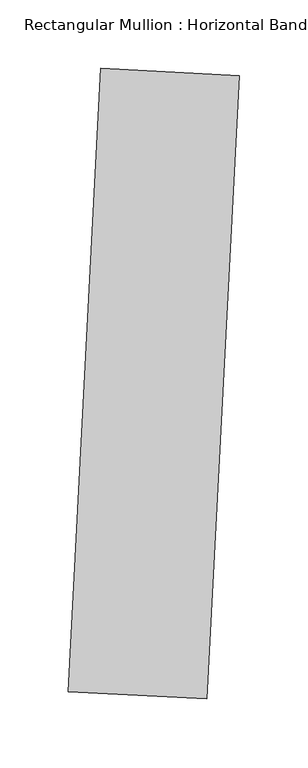
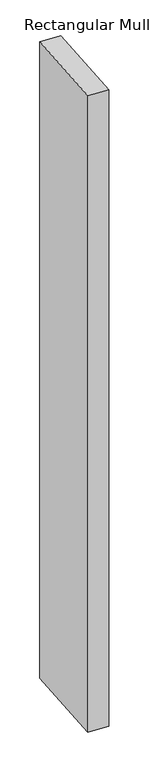
"""IFC4 building model written with IfcOpenShell, lengths in millimetres: member geometry, Rectangular Mullion : Horizontal Band."""

import ifcopenshell
import ifcopenshell.guid

model = None  # the IFC model being written
_history = None  # IfcOwnerHistory: only IFC2X3 demands one
_inside = {}  # id of a spatial element -> (the spatial element, [elements in it])
_under = {}  # id of a project, library or spatial element -> (it, [spatial elements below it])
_declared = {}  # id of a project -> (the project, [libraries it declares])
_typed = {}  # id of a type object -> (the type object, [elements of that type])
_made_of = {}  # id of a material, layer set ... -> (it, [elements and type objects made of it])


def new_model(schema):
    """Start an empty IFC model of exactly this schema.

    Asked for "IFC4X3", IfcOpenShell would pick the latest addendum, in which some entities
    have other attributes; the version numbers below select the first issue.
    IFC2X3 requires an IfcOwnerHistory on every rooted entity: one is made here for all.
    """
    global model, _history
    if schema == "IFC4X3":
        model = ifcopenshell.file(schema_version=(4, 3, 0, 0))
    else:
        model = ifcopenshell.file(schema=schema)
    _inside.clear()
    _under.clear()
    _declared.clear()
    _typed.clear()
    _made_of.clear()
    _history = None
    if model.schema == "IFC2X3":
        org = make("IfcOrganization", Name="unknown")
        user = make(
            "IfcPersonAndOrganization",
            ThePerson=make("IfcPerson", FamilyName="unknown"),
            TheOrganization=org,
        )
        app = make(
            "IfcApplication",
            ApplicationDeveloper=org,
            Version="unknown",
            ApplicationFullName="unknown",
            ApplicationIdentifier="unknown",
        )
        _history = make(
            "IfcOwnerHistory",
            OwningUser=user,
            OwningApplication=app,
            ChangeAction="ADDED",
            CreationDate=0,
        )
    return model


def make(cls, **values):
    """One entity of the class cls with the attributes given. An attribute that is None is left unset."""
    return model.create_entity(
        cls, **{name: value for name, value in values.items() if value is not None}
    )


def rooted(cls, **values):
    """An entity with a GlobalId (a new one), such as an element, a storey or a relation."""
    return make(cls, GlobalId=ifcopenshell.guid.new(), OwnerHistory=_history, **values)


def si_unit(unit_type, name, prefix=None):
    """IfcSIUnit, for example si_unit("LENGTHUNIT", "METRE", prefix="MILLI")."""
    return make("IfcSIUnit", UnitType=unit_type, Prefix=prefix, Name=name)


def assignment(units):
    """IfcUnitAssignment: the units of a project."""
    return None if units is None else make("IfcUnitAssignment", Units=units)


def point(xyz):
    """IfcCartesianPoint."""
    return None if xyz is None else make("IfcCartesianPoint", Coordinates=xyz)


def direction(xyz):
    """IfcDirection."""
    return None if xyz is None else make("IfcDirection", DirectionRatios=xyz)


def frame(location, z_axis=None, x_axis=None):
    """IfcAxis2Placement3D, a coordinate frame: its origin and axes. An axis left out is left unset."""
    return make(
        "IfcAxis2Placement3D",
        Location=point(location),
        Axis=direction(z_axis),
        RefDirection=direction(x_axis),
    )


def origin():
    """The frame at (0, 0, 0) with its axes left unset."""
    return frame((0.0, 0.0, 0.0))


def place(relative_to, where):
    """IfcLocalPlacement: puts the frame where relative to a parent placement (None: the world)."""
    return make(
        "IfcLocalPlacement", PlacementRelTo=relative_to, RelativePlacement=where
    )


def context(
    kind, dimensions, precision=None, world=None, true_north=None, identifier=None
):
    """IfcGeometricRepresentationContext, for example the 3D "Model" context."""
    return make(
        "IfcGeometricRepresentationContext",
        ContextIdentifier=identifier,
        ContextType=kind,
        CoordinateSpaceDimension=dimensions,
        Precision=precision,
        WorldCoordinateSystem=world,
        TrueNorth=true_north,
    )


def project(units=None, contexts=None):
    """IfcProject with its units and contexts."""
    return rooted(
        "IfcProject",
        Name="project",
        RepresentationContexts=contexts,
        UnitsInContext=assignment(units),
    )


def spatial(cls, under=None, at=None, **own):
    """A site, building, storey or space (cls), placed at a placement, below another one or the project."""
    s = rooted(cls, ObjectPlacement=at, **own)
    if under is not None:
        _under.setdefault(under.id(), (under, []))[1].append(s)
    return s


def polyline(points):
    """IfcPolyline through the points."""
    return make("IfcPolyline", Points=[point(p) for p in points])


def outline(outer, holes=None, kind="AREA"):
    """IfcArbitraryClosedProfileDef: a profile drawn as a closed curve; with holes, ...WithVoids."""
    if holes is None:
        return make("IfcArbitraryClosedProfileDef", ProfileType=kind, OuterCurve=outer)
    return make(
        "IfcArbitraryProfileDefWithVoids",
        ProfileType=kind,
        OuterCurve=outer,
        InnerCurves=holes,
    )


def extrude(swept, where, along, depth):
    """IfcExtrudedAreaSolid: the profile swept, set in the frame where, extruded along a direction by depth."""
    return make(
        "IfcExtrudedAreaSolid",
        SweptArea=swept,
        Position=where,
        ExtrudedDirection=direction(along),
        Depth=depth,
    )


def shape(context_of_items, identifier, shape_type, items):
    """IfcShapeRepresentation: the items that make up one representation, for example the "Body"."""
    return make(
        "IfcShapeRepresentation",
        ContextOfItems=context_of_items,
        RepresentationIdentifier=identifier,
        RepresentationType=shape_type,
        Items=items,
    )


def source(mapping_origin, context_of_items, identifier, shape_type, items):
    """IfcRepresentationMap: a shape defined once, which mapped items show again and again."""
    return make(
        "IfcRepresentationMap",
        MappingOrigin=mapping_origin,
        MappedRepresentation=shape(context_of_items, identifier, shape_type, items),
    )


def transform(
    local_origin,
    x_axis=None,
    y_axis=None,
    z_axis=None,
    scale=None,
    scale2=None,
    scale3=None,
    uniform=True,
):
    """IfcCartesianTransformationOperator3D, or its non-uniform kind. x_axis, y_axis, z_axis: its Axis1, 2, 3."""
    if uniform:
        return make(
            "IfcCartesianTransformationOperator3D",
            Axis1=direction(x_axis),
            Axis2=direction(y_axis),
            LocalOrigin=point(local_origin),
            Scale=scale,
            Axis3=direction(z_axis),
        )
    return make(
        "IfcCartesianTransformationOperator3DnonUniform",
        Axis1=direction(x_axis),
        Axis2=direction(y_axis),
        LocalOrigin=point(local_origin),
        Scale=scale,
        Axis3=direction(z_axis),
        Scale2=scale2,
        Scale3=scale3,
    )


def mapped(mapping_source, mapping_target):
    """IfcMappedItem: shows the shape of a source again, moved by a transform."""
    return make(
        "IfcMappedItem", MappingSource=mapping_source, MappingTarget=mapping_target
    )


def made_of(thing, what):
    """Note that an element or type object is made of a material, layer set ...; save() writes the relation."""
    if what is not None:
        _made_of.setdefault(what.id(), (what, []))[1].append(thing)
    return thing


def element(
    cls,
    number,
    at=None,
    inside=None,
    cuts=None,
    type_object=None,
    material=None,
    context=None,
    identifier="Body",
    shape_type=None,
    held_by="IfcProductDefinitionShape",
    body=None,
    shapes=None,
    **own,
):
    """One element of the class cls, such as IfcWall. Its Tag is "e" and its number.

    at: its placement. inside: the storey or other place that contains it. cuts: it is an
    opening in that element (IfcRelVoidsElement). A single representation is given by context,
    identifier, shape_type and body (its items); several are given by shapes. held_by: the class
    of the entity that holds the representations. save() writes the other relations.
    """
    e = rooted(cls, Tag="e%d" % number, ObjectPlacement=at, **own)
    if body is not None:
        shapes = [shape(context, identifier, shape_type, body)]
    if shapes is not None:
        e.Representation = make(held_by, Representations=shapes)
    if inside is not None:
        _inside.setdefault(inside.id(), (inside, []))[1].append(e)
    if cuts is not None:
        rooted(
            "IfcRelVoidsElement", RelatingBuildingElement=cuts, RelatedOpeningElement=e
        )
    if type_object is not None:
        _typed.setdefault(type_object.id(), (type_object, []))[1].append(e)
    return made_of(e, material)


def aggregate(whole, parts):
    """IfcRelAggregates: a whole, such as a stair, and the parts it consists of."""
    return rooted("IfcRelAggregates", RelatingObject=whole, RelatedObjects=parts)


def save(model, path):
    """Write the relations noted so far, then the file.

    IfcRelAggregates (storeys below a building ...), IfcRelContainedInSpatialStructure (elements
    in a storey), IfcRelDefinesByType, IfcRelAssociatesMaterial and IfcRelDeclares: one each for
    every whole, place, type object, material and project.
    """
    for whole, parts in _under.values():
        aggregate(whole, parts)
    for where, things in _inside.values():
        rooted(
            "IfcRelContainedInSpatialStructure",
            RelatedElements=things,
            RelatingStructure=where,
        )
    for kind, things in _typed.values():
        rooted("IfcRelDefinesByType", RelatedObjects=things, RelatingType=kind)
    for what, things in _made_of.values():
        rooted("IfcRelAssociatesMaterial", RelatedObjects=things, RelatingMaterial=what)
    for by, libraries in _declared.values():
        rooted("IfcRelDeclares", RelatingContext=by, RelatedDefinitions=libraries)
    model.write(path)


def rectangular_mullion_horizontal_band_591d7d7b(model_context):
    return source(origin(), model_context, "Body", "SweptSolid", [
        extrude(outline(polyline([(62.69438, 301.8280451), (38.7663808, -154.7453782), (-62.69438, -149.4280451), (-38.7663808, 307.1453782), (62.69438, 301.8280451)])), frame((0.0, 0.0, -3352.8), z_axis=(0.0, 0.0, 1.0), x_axis=(1.0, 0.0, 0.0)), (0.0, 0.0, 1.0), 3352.8),
    ])


if __name__ == "__main__":
    model = new_model("IFC4")
    model_context = context("Model", 3, world=origin())
    ifc_project = project(units=[si_unit("LENGTHUNIT", "METRE", prefix="MILLI")], contexts=[model_context])
    site = spatial("IfcSite", under=ifc_project)
    building = spatial("IfcBuilding", under=site)
    placement = place(None, origin())
    rectangular_mullion_horizontal_band_shape = rectangular_mullion_horizontal_band_591d7d7b(model_context)
    element("IfcMember", 1, ObjectType="Rectangular Mullion : Horizontal Band", at=placement, inside=building, context=model_context, shape_type="MappedRepresentation", body=[
        mapped(rectangular_mullion_horizontal_band_shape, transform((0.0, 0.0, 0.0), x_axis=(1.0, 0.0, 0.0), y_axis=(0.0, 1.0, 0.0), z_axis=(0.0, 0.0, 1.0))),
    ])
    save(model, "model.ifc")

# Revit data of these elements
# Type "Rectangular Mullion : Horizontal Band"
#   built-in parameter 1007351 = 0.25 (stored number, unit not read)
#   built-in parameter 1007304 = 1.5 (stored number, unit not read)
#   built-in parameter 1007301 = 0.166667 (stored number, unit not read)
#   built-in parameter 1007300 = 0.166667 (stored number, unit not read)
# Element 1 (IfcMember, "Rectangular Mullion : Horizontal Band")
#   Materials on its faces: "Aluminum"
# Materials
#   "Aluminum": class "Metal", colour RGB 247 247 247, transparency 0, Description = "Aluminum 6061", Cost = 0
